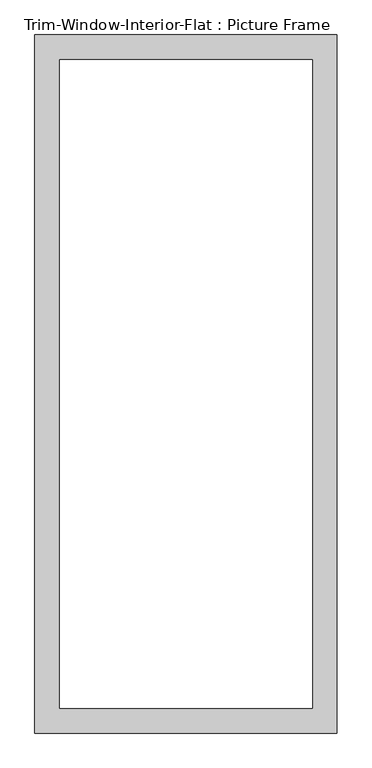
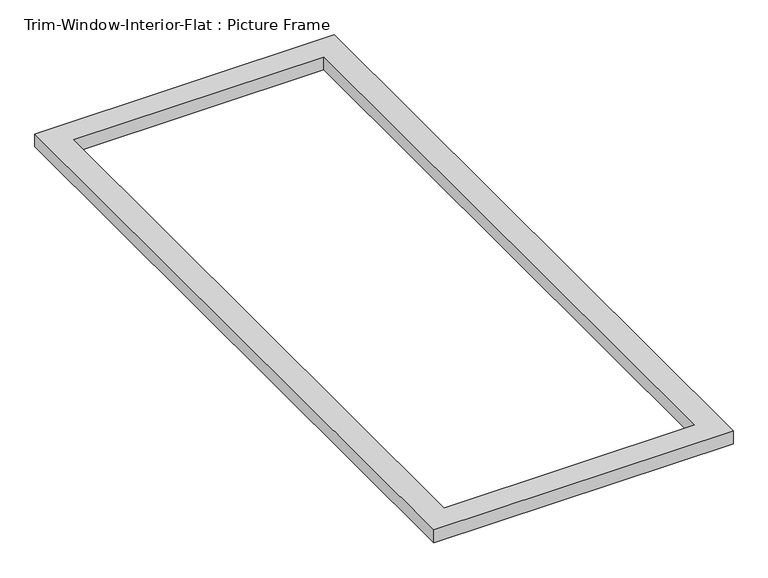
"""IFC4 building model written with IfcOpenShell, lengths in millimetres: proxy geometry, Trim-Window-Interior-Flat : Picture Frame."""

import ifcopenshell
import ifcopenshell.guid

model = None  # the IFC model being written
_history = None  # IfcOwnerHistory: only IFC2X3 demands one
_inside = {}  # id of a spatial element -> (the spatial element, [elements in it])
_under = {}  # id of a project, library or spatial element -> (it, [spatial elements below it])
_declared = {}  # id of a project -> (the project, [libraries it declares])
_typed = {}  # id of a type object -> (the type object, [elements of that type])
_made_of = {}  # id of a material, layer set ... -> (it, [elements and type objects made of it])


def new_model(schema):
    """Start an empty IFC model of exactly this schema.

    Asked for "IFC4X3", IfcOpenShell would pick the latest addendum, in which some entities
    have other attributes; the version numbers below select the first issue.
    IFC2X3 requires an IfcOwnerHistory on every rooted entity: one is made here for all.
    """
    global model, _history
    if schema == "IFC4X3":
        model = ifcopenshell.file(schema_version=(4, 3, 0, 0))
    else:
        model = ifcopenshell.file(schema=schema)
    _inside.clear()
    _under.clear()
    _declared.clear()
    _typed.clear()
    _made_of.clear()
    _history = None
    if model.schema == "IFC2X3":
        org = make("IfcOrganization", Name="unknown")
        user = make(
            "IfcPersonAndOrganization",
            ThePerson=make("IfcPerson", FamilyName="unknown"),
            TheOrganization=org,
        )
        app = make(
            "IfcApplication",
            ApplicationDeveloper=org,
            Version="unknown",
            ApplicationFullName="unknown",
            ApplicationIdentifier="unknown",
        )
        _history = make(
            "IfcOwnerHistory",
            OwningUser=user,
            OwningApplication=app,
            ChangeAction="ADDED",
            CreationDate=0,
        )
    return model


def make(cls, **values):
    """One entity of the class cls with the attributes given. An attribute that is None is left unset."""
    return model.create_entity(
        cls, **{name: value for name, value in values.items() if value is not None}
    )


def rooted(cls, **values):
    """An entity with a GlobalId (a new one), such as an element, a storey or a relation."""
    return make(cls, GlobalId=ifcopenshell.guid.new(), OwnerHistory=_history, **values)


def si_unit(unit_type, name, prefix=None):
    """IfcSIUnit, for example si_unit("LENGTHUNIT", "METRE", prefix="MILLI")."""
    return make("IfcSIUnit", UnitType=unit_type, Prefix=prefix, Name=name)


def assignment(units):
    """IfcUnitAssignment: the units of a project."""
    return None if units is None else make("IfcUnitAssignment", Units=units)


def point(xyz):
    """IfcCartesianPoint."""
    return None if xyz is None else make("IfcCartesianPoint", Coordinates=xyz)


def direction(xyz):
    """IfcDirection."""
    return None if xyz is None else make("IfcDirection", DirectionRatios=xyz)


def frame(location, z_axis=None, x_axis=None):
    """IfcAxis2Placement3D, a coordinate frame: its origin and axes. An axis left out is left unset."""
    return make(
        "IfcAxis2Placement3D",
        Location=point(location),
        Axis=direction(z_axis),
        RefDirection=direction(x_axis),
    )


def origin():
    """The frame at (0, 0, 0) with its axes left unset."""
    return frame((0.0, 0.0, 0.0))


def origin_with_axes():
    """The frame at (0, 0, 0) with the z axis (0, 0, 1) and the x axis (1, 0, 0) written out."""
    return frame((0.0, 0.0, 0.0), z_axis=(0.0, 0.0, 1.0), x_axis=(1.0, 0.0, 0.0))


def place(relative_to, where):
    """IfcLocalPlacement: puts the frame where relative to a parent placement (None: the world)."""
    return make(
        "IfcLocalPlacement", PlacementRelTo=relative_to, RelativePlacement=where
    )


def context(
    kind, dimensions, precision=None, world=None, true_north=None, identifier=None
):
    """IfcGeometricRepresentationContext, for example the 3D "Model" context."""
    return make(
        "IfcGeometricRepresentationContext",
        ContextIdentifier=identifier,
        ContextType=kind,
        CoordinateSpaceDimension=dimensions,
        Precision=precision,
        WorldCoordinateSystem=world,
        TrueNorth=true_north,
    )


def project(units=None, contexts=None):
    """IfcProject with its units and contexts."""
    return rooted(
        "IfcProject",
        Name="project",
        RepresentationContexts=contexts,
        UnitsInContext=assignment(units),
    )


def spatial(cls, under=None, at=None, **own):
    """A site, building, storey or space (cls), placed at a placement, below another one or the project."""
    s = rooted(cls, ObjectPlacement=at, **own)
    if under is not None:
        _under.setdefault(under.id(), (under, []))[1].append(s)
    return s


def polyline(points):
    """IfcPolyline through the points."""
    return make("IfcPolyline", Points=[point(p) for p in points])


def outline(outer, holes=None, kind="AREA"):
    """IfcArbitraryClosedProfileDef: a profile drawn as a closed curve; with holes, ...WithVoids."""
    if holes is None:
        return make("IfcArbitraryClosedProfileDef", ProfileType=kind, OuterCurve=outer)
    return make(
        "IfcArbitraryProfileDefWithVoids",
        ProfileType=kind,
        OuterCurve=outer,
        InnerCurves=holes,
    )


def extrude(swept, where, along, depth):
    """IfcExtrudedAreaSolid: the profile swept, set in the frame where, extruded along a direction by depth."""
    return make(
        "IfcExtrudedAreaSolid",
        SweptArea=swept,
        Position=where,
        ExtrudedDirection=direction(along),
        Depth=depth,
    )


def shape(context_of_items, identifier, shape_type, items):
    """IfcShapeRepresentation: the items that make up one representation, for example the "Body"."""
    return make(
        "IfcShapeRepresentation",
        ContextOfItems=context_of_items,
        RepresentationIdentifier=identifier,
        RepresentationType=shape_type,
        Items=items,
    )


def source(mapping_origin, context_of_items, identifier, shape_type, items):
    """IfcRepresentationMap: a shape defined once, which mapped items show again and again."""
    return make(
        "IfcRepresentationMap",
        MappingOrigin=mapping_origin,
        MappedRepresentation=shape(context_of_items, identifier, shape_type, items),
    )


def transform(
    local_origin,
    x_axis=None,
    y_axis=None,
    z_axis=None,
    scale=None,
    scale2=None,
    scale3=None,
    uniform=True,
):
    """IfcCartesianTransformationOperator3D, or its non-uniform kind. x_axis, y_axis, z_axis: its Axis1, 2, 3."""
    if uniform:
        return make(
            "IfcCartesianTransformationOperator3D",
            Axis1=direction(x_axis),
            Axis2=direction(y_axis),
            LocalOrigin=point(local_origin),
            Scale=scale,
            Axis3=direction(z_axis),
        )
    return make(
        "IfcCartesianTransformationOperator3DnonUniform",
        Axis1=direction(x_axis),
        Axis2=direction(y_axis),
        LocalOrigin=point(local_origin),
        Scale=scale,
        Axis3=direction(z_axis),
        Scale2=scale2,
        Scale3=scale3,
    )


def mapped(mapping_source, mapping_target):
    """IfcMappedItem: shows the shape of a source again, moved by a transform."""
    return make(
        "IfcMappedItem", MappingSource=mapping_source, MappingTarget=mapping_target
    )


def made_of(thing, what):
    """Note that an element or type object is made of a material, layer set ...; save() writes the relation."""
    if what is not None:
        _made_of.setdefault(what.id(), (what, []))[1].append(thing)
    return thing


def element(
    cls,
    number,
    at=None,
    inside=None,
    cuts=None,
    type_object=None,
    material=None,
    context=None,
    identifier="Body",
    shape_type=None,
    held_by="IfcProductDefinitionShape",
    body=None,
    shapes=None,
    **own,
):
    """One element of the class cls, such as IfcWall. Its Tag is "e" and its number.

    at: its placement. inside: the storey or other place that contains it. cuts: it is an
    opening in that element (IfcRelVoidsElement). A single representation is given by context,
    identifier, shape_type and body (its items); several are given by shapes. held_by: the class
    of the entity that holds the representations. save() writes the other relations.
    """
    e = rooted(cls, Tag="e%d" % number, ObjectPlacement=at, **own)
    if body is not None:
        shapes = [shape(context, identifier, shape_type, body)]
    if shapes is not None:
        e.Representation = make(held_by, Representations=shapes)
    if inside is not None:
        _inside.setdefault(inside.id(), (inside, []))[1].append(e)
    if cuts is not None:
        rooted(
            "IfcRelVoidsElement", RelatingBuildingElement=cuts, RelatedOpeningElement=e
        )
    if type_object is not None:
        _typed.setdefault(type_object.id(), (type_object, []))[1].append(e)
    return made_of(e, material)


def aggregate(whole, parts):
    """IfcRelAggregates: a whole, such as a stair, and the parts it consists of."""
    return rooted("IfcRelAggregates", RelatingObject=whole, RelatedObjects=parts)


def save(model, path):
    """Write the relations noted so far, then the file.

    IfcRelAggregates (storeys below a building ...), IfcRelContainedInSpatialStructure (elements
    in a storey), IfcRelDefinesByType, IfcRelAssociatesMaterial and IfcRelDeclares: one each for
    every whole, place, type object, material and project.
    """
    for whole, parts in _under.values():
        aggregate(whole, parts)
    for where, things in _inside.values():
        rooted(
            "IfcRelContainedInSpatialStructure",
            RelatedElements=things,
            RelatingStructure=where,
        )
    for kind, things in _typed.values():
        rooted("IfcRelDefinesByType", RelatedObjects=things, RelatingType=kind)
    for what, things in _made_of.values():
        rooted("IfcRelAssociatesMaterial", RelatedObjects=things, RelatingMaterial=what)
    for by, libraries in _declared.values():
        rooted("IfcRelDeclares", RelatingContext=by, RelatedDefinitions=libraries)
    model.write(path)


def trim_window_interior_flat_picture_frame_978fd00d(model_context):
    return source(origin(), model_context, "Body", "SweptSolid", [
        extrude(outline(polyline([(349.25, 44.45), (349.25, -1568.45), (-349.25, -1568.45), (-349.25, 44.45), (349.25, 44.45)]), holes=[polyline([(292.1, -12.7), (-292.1, -12.7), (-292.1, -1511.3), (292.1, -1511.3), (292.1, -12.7)])]), origin_with_axes(), (0.0, 0.0, 1.0), 31.75),
    ])


if __name__ == "__main__":
    model = new_model("IFC4")
    model_context = context("Model", 3, world=origin())
    ifc_project = project(units=[si_unit("LENGTHUNIT", "METRE", prefix="MILLI")], contexts=[model_context])
    site = spatial("IfcSite", under=ifc_project)
    building = spatial("IfcBuilding", under=site)
    placement = place(None, origin())
    trim_window_interior_flat_picture_frame_shape = trim_window_interior_flat_picture_frame_978fd00d(model_context)
    element("IfcBuildingElementProxy", 1, Name="Trim-Window-Interior-Flat : Picture Frame", ObjectType="Trim-Window-Interior-Flat : Picture Frame", at=placement, inside=building, context=model_context, shape_type="MappedRepresentation", body=[
        mapped(trim_window_interior_flat_picture_frame_shape, transform((0.0, 0.0, 0.0), x_axis=(1.0, 0.0, 0.0), y_axis=(0.0, 1.0, 0.0), z_axis=(0.0, 0.0, 1.0))),
    ])
    save(model, "model.ifc")

# Revit data of these elements
# Type "Trim-Window-Interior-Flat : Picture Frame"
#   Trim Thickness_Picture Frame = 0' - 1 1/4"
#   Trim Width = 0' - 2 1/4"
#   Trim Thickness_with Sill = 0' - 0 3/4"
#   Sill Thickness = 0' - 1 1/4"
#   Opening Width [instance default] = 2' - 0"
#   Opening Height [instance default] = 3' - 0"
#   Default Elevation = 4' - 0"
#   Sill = no
#   Picture Frame = yes
#   Trim Material [instance default] = none
# Element 1 (IfcBuildingElementProxy, "Trim-Window-Interior-Flat : Picture Frame")
#   Opening Height = 5' - 0"
#   Trim Material = Wood - Stained
#   Materials on its faces: "Wood - Stained"
# Materials
#   "Wood - Stained": class "Wood", colour RGB 224 178 126, transparency 0, Cost = 0
